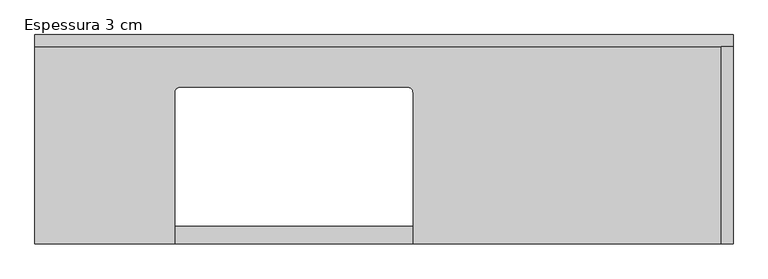
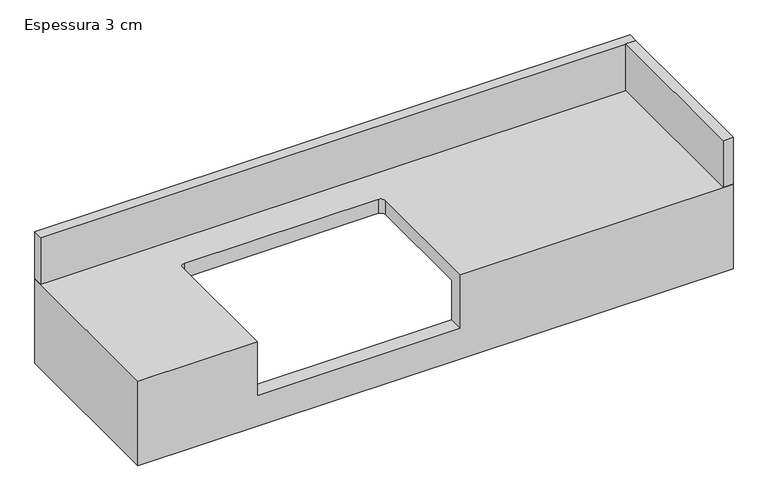
"""IFC4 building model written with IfcOpenShell, lengths in millimetres: furniture geometry, CC_BANCADA BANHEIRO COM CUBA_CANTO RETO : Espessura 3 cm."""

from ifc_helpers import new_model, si_unit, frame, origin, place, context, project, spatial, polyline, circle_curve, outline, extrude, source, transform, mapped, element, save
from ifc_brep_helpers import plane_surface, revolved_surface, advanced_brep


def espessura_3_cm_9ecbce42(model_context):
    return source(origin(), model_context, "Body", "SolidModel", [
        advanced_brep(
        [(750.0, 300.0, 860.0), (-450.0, 300.0, 860.0), (-450.0, -60.0, 860.0), (-210.0, -60.0, 860.0), (-210.0, 200.0, 860.0), (-200.0, 210.0, 860.0), (190.0, 210.0, 860.0), (200.0, 200.0, 860.0), (200.0, -60.0, 860.0), (750.0, -60.0, 860.0), (750.0, 300.0, 680.0), (720.0, 300.0, 680.0), (720.0, 300.0, 830.0), (-420.0, 300.0, 830.0), (-420.0, 300.0, 680.0), (-450.0, 300.0, 680.0), (-450.0, -60.0, 680.0), (750.0, -60.0, 680.0), (200.0, -60.0, 745.0), (-210.0, -60.0, 745.0), (720.0, -30.0, 830.0), (200.0, -30.0, 830.0), (200.0, 200.0, 830.0), (190.0, 210.0, 830.0), (-200.0, 210.0, 830.0), (-210.0, 200.0, 830.0), (-210.0, -30.0, 830.0), (-420.0, -30.0, 830.0), (-420.0, -30.0, 680.0), (-210.0, -30.0, 745.0), (200.0, -30.0, 745.0), (720.0, -30.0, 680.0)],
        [
            (0, 1),
            (1, 2),
            (2, 3),
            (3, 4),
            (4, 5, circle_curve(frame((-200.0, 200.0, 860.0), z_axis=(0.0, 0.0, -1.0), x_axis=(0.0, 1.0, 0.0)), 10.0)),
            (5, 6),
            (6, 7, circle_curve(frame((190.0, 200.0, 860.0), z_axis=(0.0, 0.0, -1.0), x_axis=(0.0, 1.0, 0.0)), 10.0)),
            (7, 8),
            (8, 9),
            (9, 0),
            (0, 10),
            (10, 11),
            (11, 12),
            (12, 13),
            (13, 14),
            (14, 15),
            (15, 1),
            (15, 16),
            (16, 2),
            (16, 17),
            (17, 9),
            (8, 18),
            (18, 19),
            (19, 3),
            (17, 10),
            (12, 20),
            (20, 21),
            (21, 22),
            (22, 23, circle_curve(frame((190.0, 200.0, 830.0), z_axis=(0.0, 0.0, 1.0), x_axis=(0.0, 1.0, 0.0)), 10.0)),
            (23, 24),
            (24, 25, circle_curve(frame((-200.0, 200.0, 830.0), z_axis=(0.0, 0.0, 1.0), x_axis=(0.0, 1.0, 0.0)), 10.0)),
            (25, 26),
            (26, 27),
            (27, 13),
            (27, 28),
            (28, 14),
            (26, 29),
            (29, 30),
            (30, 21),
            (20, 31),
            (31, 28),
            (11, 31),
            (5, 24),
            (23, 6),
            (18, 30),
            (29, 19),
            (4, 25),
            (7, 22),
        ],
        [
            plane_surface(frame((-450.0, 300.0, 860.0), z_axis=(0.0, 0.0, 1.0), x_axis=(-1.0, 0.0, 0.0))),
            plane_surface(frame((750.0, 300.0, 860.0), z_axis=(0.0, 1.0, 0.0), x_axis=(0.0, 0.0, -1.0))),
            plane_surface(frame((-450.0, 300.0, 860.0), z_axis=(-1.0, 0.0, 0.0), x_axis=(0.0, 0.0, -1.0))),
            plane_surface(frame((-450.0, -60.0, 860.0), z_axis=(0.0, -1.0, 0.0), x_axis=(0.0, 0.0, -1.0))),
            plane_surface(frame((750.0, -60.0, 860.0), z_axis=(1.0, 0.0, 0.0), x_axis=(0.0, 0.0, -1.0))),
            plane_surface(frame((-420.0, 300.0, 830.0), z_axis=(0.0, 0.0, -1.0), x_axis=(-1.0, 0.0, 0.0))),
            plane_surface(frame((-420.0, 300.0, 830.0), z_axis=(1.0, 0.0, 0.0), x_axis=(0.0, 0.0, -1.0))),
            plane_surface(frame((-420.0, -30.0, 830.0), z_axis=(0.0, 1.0, 0.0), x_axis=(0.0, 0.0, -1.0))),
            plane_surface(frame((720.0, -30.0, 830.0), z_axis=(-1.0, 0.0, 0.0), x_axis=(0.0, 0.0, -1.0))),
            plane_surface(frame((750.0, -60.0, 680.0), z_axis=(0.0, 0.0, -1.0), x_axis=(0.0, 1.0, 0.0))),
            plane_surface(frame((-200.0, 210.0, 745.0), z_axis=(0.0, -1.0, 0.0), x_axis=(0.0, 0.0, 1.0))),
            plane_surface(frame((190.0, 210.0, 745.0), z_axis=(0.0, 0.0, 1.0), x_axis=(1.0, 0.0, 0.0))),
            revolved_surface(polyline([(-200.0, 210.0, 830.0), (-200.0, 210.0, 860.0)]), (-200.0, 200.0, 900.0), (0.0, 0.0, -1.0)),
            plane_surface(frame((-210.0, -190.0, 745.0), z_axis=(1.0, 0.0, 0.0), x_axis=(0.0, 0.0, 1.0))),
            plane_surface(frame((200.0, 200.0, 745.0), z_axis=(-1.0, 0.0, 0.0), x_axis=(0.0, 0.0, 1.0))),
            revolved_surface(polyline([(190.0, 210.0, 830.0), (190.0, 210.0, 860.0)]), (190.0, 200.0, 900.0), (0.0, 0.0, -1.0)),
        ],
        [
            (0, [[1, 2, 3, 4, 5, 6, 7, 8, 9, 10]]),
            (1, [[-1, 11, 12, 13, 14, 15, 16, 17]]),
            (2, [[-2, -17, 18, 19]]),
            (3, [[-3, -19, 20, 21, -9, 22, 23, 24]]),
            (4, [[-10, -21, 25, -11]]),
            (5, [[26, 27, 28, 29, 30, 31, 32, 33, 34, -14]]),
            (6, [[-34, 35, 36, -15]]),
            (7, [[-33, 37, 38, 39, -27, 40, 41, -35]]),
            (8, [[-26, -13, 42, -40]]),
            (9, [[-12, -25, -20, -18, -16, -36, -41, -42]]),
            (10, [[-6, 43, -30, 44]]),
            (11, [[-23, 45, -38, 46]]),
            (12, [[-5, 47, -31, -43]]),
            (13, [[-4, -24, -46, -37, -32, -47]]),
            (14, [[-8, 48, -28, -39, -45, -22]]),
            (15, [[-7, -44, -29, -48]]),
        ],
    ),
        extrude(outline(polyline([(730.0, 280.0), (750.0, 280.0), (750.0, -60.0), (730.0, -60.0), (730.0, 280.0)])), frame((0.0, 0.0, 860.0), z_axis=(0.0, 0.0, 1.0), x_axis=(1.0, 0.0, 0.0)), (0.0, 0.0, 1.0), 100.0),
        extrude(outline(polyline([(750.0, 300.0), (750.0, 280.0), (-450.0, 280.0), (-450.0, 300.0), (750.0, 300.0)])), frame((0.0, 0.0, 860.0), z_axis=(0.0, 0.0, 1.0), x_axis=(1.0, 0.0, 0.0)), (0.0, 0.0, 1.0), 100.0),
    ])


if __name__ == "__main__":
    model = new_model("IFC4")
    model_context = context("Model", 3, world=origin())
    ifc_project = project(units=[si_unit("LENGTHUNIT", "METRE", prefix="MILLI")], contexts=[model_context])
    site = spatial("IfcSite", under=ifc_project)
    building = spatial("IfcBuilding", under=site)
    placement = place(None, origin())
    espessura_3_cm_shape = espessura_3_cm_9ecbce42(model_context)
    element("IfcFurniture", 1, ObjectType="CC_BANCADA BANHEIRO COM CUBA_CANTO RETO : Espessura 3 cm", at=placement, inside=building, context=model_context, shape_type="MappedRepresentation", body=[
        mapped(espessura_3_cm_shape, transform((0.0, 0.0, 0.0), x_axis=(1.0, 0.0, 0.0), y_axis=(0.0, 1.0, 0.0), z_axis=(0.0, 0.0, 1.0))),
    ])
    save(model, "model.ifc")

# Revit data of these elements
# Type "CC_BANCADA BANHEIRO COM CUBA_CANTO RETO : Espessura 3 cm"
#   Uso HS [instance default] = ""
#   h TESTEIRA AUX [instance default] = 0.15 m
#   Altura testeira [instance default] = 0.15 m
#   Altura rodapia [instance default] = 0.10 m
#   Espessura rodapia [instance default] = 0.02 m
#   Prof/2 [instance default] = 0.20 m
#   Offset cuba esquerda [instance default] = 0.40 m
#   Depth [instance default] = 1.20 m
#   Width [instance default] = 0.40 m
#   Espessura bancada = 0.03 m
#   Comprimento [instance default] = 1.20 m
#   Height [instance default] = 0.86 m
#   Testeira [instance default] = yes
#   Rodapia fundo [instance default] = no
#   Rodapia esquerda [instance default] = no
#   Rodapia direita [instance default] = no
#   Material porta-toalha [instance default] = .CROMADO
#   Material hidráulico [instance default] = .CROMADO
#   Material cuba [instance default] = .PORCELANA BRANCA
#   Material bancada [instance default] = .GRANITO_BRANCO_ITAUNAS
#   Assembly Code = ""
# Element 1 (IfcFurniture, "CC_BANCADA BANHEIRO COM CUBA_CANTO RETO : Espessura 3 cm")
#   Uso HS = "VESTIÁRIO"
#   Prof/2 = 0.18 m
#   Offset cuba esquerda = 0.24 m
#   Width = 0.36 m
#   Rodapia fundo = yes
#   Rodapia direita = yes
#   Materials on its faces: ".GRANITO_BRANCO_ITAUNAS"
# Materials
#   ".CROMADO": class "CC_METAIS", colour RGB 211 223 226, transparency 0, Cost = 0
#   ".PORCELANA BRANCA": class "CC_PORCELANA", colour RGB 230 230 230, transparency 0, Cost = 0
#   ".GRANITO_BRANCO_ITAUNAS": class ".CC_PEDRA REVEST.", colour RGB 202 195 174, transparency 0, Description = "Revestimento em granito", Cost = 0
